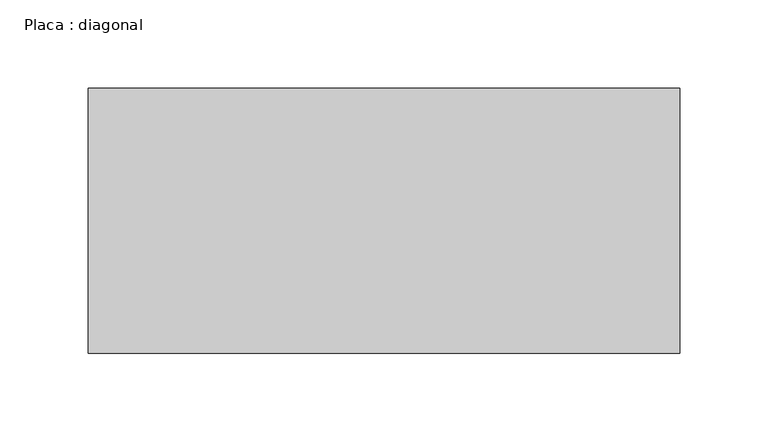
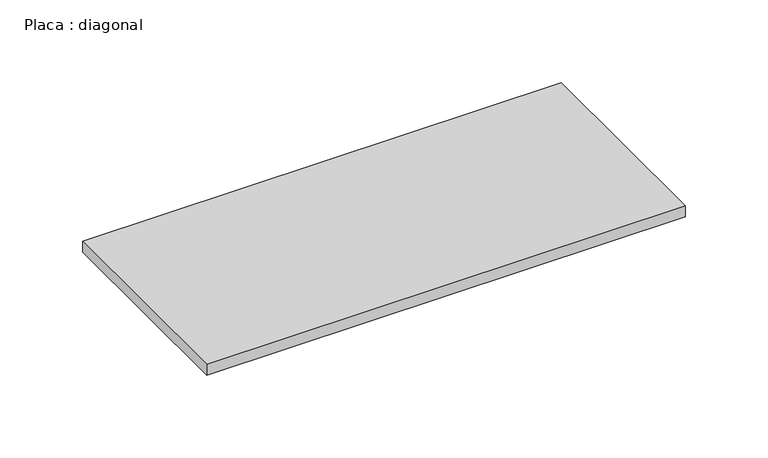
"""IFC4 building model written with IfcOpenShell, lengths in millimetres: beam geometry, Placa : diagonal."""

import ifcopenshell
import ifcopenshell.guid

model = None  # the IFC model being written
_history = None  # IfcOwnerHistory: only IFC2X3 demands one
_inside = {}  # id of a spatial element -> (the spatial element, [elements in it])
_under = {}  # id of a project, library or spatial element -> (it, [spatial elements below it])
_declared = {}  # id of a project -> (the project, [libraries it declares])
_typed = {}  # id of a type object -> (the type object, [elements of that type])
_made_of = {}  # id of a material, layer set ... -> (it, [elements and type objects made of it])


def new_model(schema):
    """Start an empty IFC model of exactly this schema.

    Asked for "IFC4X3", IfcOpenShell would pick the latest addendum, in which some entities
    have other attributes; the version numbers below select the first issue.
    IFC2X3 requires an IfcOwnerHistory on every rooted entity: one is made here for all.
    """
    global model, _history
    if schema == "IFC4X3":
        model = ifcopenshell.file(schema_version=(4, 3, 0, 0))
    else:
        model = ifcopenshell.file(schema=schema)
    _inside.clear()
    _under.clear()
    _declared.clear()
    _typed.clear()
    _made_of.clear()
    _history = None
    if model.schema == "IFC2X3":
        org = make("IfcOrganization", Name="unknown")
        user = make(
            "IfcPersonAndOrganization",
            ThePerson=make("IfcPerson", FamilyName="unknown"),
            TheOrganization=org,
        )
        app = make(
            "IfcApplication",
            ApplicationDeveloper=org,
            Version="unknown",
            ApplicationFullName="unknown",
            ApplicationIdentifier="unknown",
        )
        _history = make(
            "IfcOwnerHistory",
            OwningUser=user,
            OwningApplication=app,
            ChangeAction="ADDED",
            CreationDate=0,
        )
    return model


def make(cls, **values):
    """One entity of the class cls with the attributes given. An attribute that is None is left unset."""
    return model.create_entity(
        cls, **{name: value for name, value in values.items() if value is not None}
    )


def rooted(cls, **values):
    """An entity with a GlobalId (a new one), such as an element, a storey or a relation."""
    return make(cls, GlobalId=ifcopenshell.guid.new(), OwnerHistory=_history, **values)


def si_unit(unit_type, name, prefix=None):
    """IfcSIUnit, for example si_unit("LENGTHUNIT", "METRE", prefix="MILLI")."""
    return make("IfcSIUnit", UnitType=unit_type, Prefix=prefix, Name=name)


def assignment(units):
    """IfcUnitAssignment: the units of a project."""
    return None if units is None else make("IfcUnitAssignment", Units=units)


def point(xyz):
    """IfcCartesianPoint."""
    return None if xyz is None else make("IfcCartesianPoint", Coordinates=xyz)


def direction(xyz):
    """IfcDirection."""
    return None if xyz is None else make("IfcDirection", DirectionRatios=xyz)


def frame(location, z_axis=None, x_axis=None):
    """IfcAxis2Placement3D, a coordinate frame: its origin and axes. An axis left out is left unset."""
    return make(
        "IfcAxis2Placement3D",
        Location=point(location),
        Axis=direction(z_axis),
        RefDirection=direction(x_axis),
    )


def origin():
    """The frame at (0, 0, 0) with its axes left unset."""
    return frame((0.0, 0.0, 0.0))


def place(relative_to, where):
    """IfcLocalPlacement: puts the frame where relative to a parent placement (None: the world)."""
    return make(
        "IfcLocalPlacement", PlacementRelTo=relative_to, RelativePlacement=where
    )


def context(
    kind, dimensions, precision=None, world=None, true_north=None, identifier=None
):
    """IfcGeometricRepresentationContext, for example the 3D "Model" context."""
    return make(
        "IfcGeometricRepresentationContext",
        ContextIdentifier=identifier,
        ContextType=kind,
        CoordinateSpaceDimension=dimensions,
        Precision=precision,
        WorldCoordinateSystem=world,
        TrueNorth=true_north,
    )


def project(units=None, contexts=None):
    """IfcProject with its units and contexts."""
    return rooted(
        "IfcProject",
        Name="project",
        RepresentationContexts=contexts,
        UnitsInContext=assignment(units),
    )


def spatial(cls, under=None, at=None, **own):
    """A site, building, storey or space (cls), placed at a placement, below another one or the project."""
    s = rooted(cls, ObjectPlacement=at, **own)
    if under is not None:
        _under.setdefault(under.id(), (under, []))[1].append(s)
    return s


def polyline(points):
    """IfcPolyline through the points."""
    return make("IfcPolyline", Points=[point(p) for p in points])


def outline(outer, holes=None, kind="AREA"):
    """IfcArbitraryClosedProfileDef: a profile drawn as a closed curve; with holes, ...WithVoids."""
    if holes is None:
        return make("IfcArbitraryClosedProfileDef", ProfileType=kind, OuterCurve=outer)
    return make(
        "IfcArbitraryProfileDefWithVoids",
        ProfileType=kind,
        OuterCurve=outer,
        InnerCurves=holes,
    )


def extrude(swept, where, along, depth):
    """IfcExtrudedAreaSolid: the profile swept, set in the frame where, extruded along a direction by depth."""
    return make(
        "IfcExtrudedAreaSolid",
        SweptArea=swept,
        Position=where,
        ExtrudedDirection=direction(along),
        Depth=depth,
    )


def shape(context_of_items, identifier, shape_type, items):
    """IfcShapeRepresentation: the items that make up one representation, for example the "Body"."""
    return make(
        "IfcShapeRepresentation",
        ContextOfItems=context_of_items,
        RepresentationIdentifier=identifier,
        RepresentationType=shape_type,
        Items=items,
    )


def source(mapping_origin, context_of_items, identifier, shape_type, items):
    """IfcRepresentationMap: a shape defined once, which mapped items show again and again."""
    return make(
        "IfcRepresentationMap",
        MappingOrigin=mapping_origin,
        MappedRepresentation=shape(context_of_items, identifier, shape_type, items),
    )


def transform(
    local_origin,
    x_axis=None,
    y_axis=None,
    z_axis=None,
    scale=None,
    scale2=None,
    scale3=None,
    uniform=True,
):
    """IfcCartesianTransformationOperator3D, or its non-uniform kind. x_axis, y_axis, z_axis: its Axis1, 2, 3."""
    if uniform:
        return make(
            "IfcCartesianTransformationOperator3D",
            Axis1=direction(x_axis),
            Axis2=direction(y_axis),
            LocalOrigin=point(local_origin),
            Scale=scale,
            Axis3=direction(z_axis),
        )
    return make(
        "IfcCartesianTransformationOperator3DnonUniform",
        Axis1=direction(x_axis),
        Axis2=direction(y_axis),
        LocalOrigin=point(local_origin),
        Scale=scale,
        Axis3=direction(z_axis),
        Scale2=scale2,
        Scale3=scale3,
    )


def mapped(mapping_source, mapping_target):
    """IfcMappedItem: shows the shape of a source again, moved by a transform."""
    return make(
        "IfcMappedItem", MappingSource=mapping_source, MappingTarget=mapping_target
    )


def made_of(thing, what):
    """Note that an element or type object is made of a material, layer set ...; save() writes the relation."""
    if what is not None:
        _made_of.setdefault(what.id(), (what, []))[1].append(thing)
    return thing


def element(
    cls,
    number,
    at=None,
    inside=None,
    cuts=None,
    type_object=None,
    material=None,
    context=None,
    identifier="Body",
    shape_type=None,
    held_by="IfcProductDefinitionShape",
    body=None,
    shapes=None,
    **own,
):
    """One element of the class cls, such as IfcWall. Its Tag is "e" and its number.

    at: its placement. inside: the storey or other place that contains it. cuts: it is an
    opening in that element (IfcRelVoidsElement). A single representation is given by context,
    identifier, shape_type and body (its items); several are given by shapes. held_by: the class
    of the entity that holds the representations. save() writes the other relations.
    """
    e = rooted(cls, Tag="e%d" % number, ObjectPlacement=at, **own)
    if body is not None:
        shapes = [shape(context, identifier, shape_type, body)]
    if shapes is not None:
        e.Representation = make(held_by, Representations=shapes)
    if inside is not None:
        _inside.setdefault(inside.id(), (inside, []))[1].append(e)
    if cuts is not None:
        rooted(
            "IfcRelVoidsElement", RelatingBuildingElement=cuts, RelatedOpeningElement=e
        )
    if type_object is not None:
        _typed.setdefault(type_object.id(), (type_object, []))[1].append(e)
    return made_of(e, material)


def aggregate(whole, parts):
    """IfcRelAggregates: a whole, such as a stair, and the parts it consists of."""
    return rooted("IfcRelAggregates", RelatingObject=whole, RelatedObjects=parts)


def save(model, path):
    """Write the relations noted so far, then the file.

    IfcRelAggregates (storeys below a building ...), IfcRelContainedInSpatialStructure (elements
    in a storey), IfcRelDefinesByType, IfcRelAssociatesMaterial and IfcRelDeclares: one each for
    every whole, place, type object, material and project.
    """
    for whole, parts in _under.values():
        aggregate(whole, parts)
    for where, things in _inside.values():
        rooted(
            "IfcRelContainedInSpatialStructure",
            RelatedElements=things,
            RelatingStructure=where,
        )
    for kind, things in _typed.values():
        rooted("IfcRelDefinesByType", RelatedObjects=things, RelatingType=kind)
    for what, things in _made_of.values():
        rooted("IfcRelAssociatesMaterial", RelatedObjects=things, RelatingMaterial=what)
    for by, libraries in _declared.values():
        rooted("IfcRelDeclares", RelatingContext=by, RelatedDefinitions=libraries)
    model.write(path)


def placa_diagonal_266b1673(model_context):
    return source(origin(), model_context, "Body", "SweptSolid", [
        extrude(outline(polyline([(167.1833817, 75.0), (167.1833817, -75.0), (-167.541755, -75.0), (-167.541755, 75.0), (167.1833817, 75.0)])), frame((0.0, 0.0, -4.0), z_axis=(0.0, 0.0, 1.0), x_axis=(1.0, 0.0, 0.0)), (0.0, 0.0, 1.0), 8.0),
    ])


if __name__ == "__main__":
    model = new_model("IFC4")
    model_context = context("Model", 3, world=origin())
    ifc_project = project(units=[si_unit("LENGTHUNIT", "METRE", prefix="MILLI")], contexts=[model_context])
    site = spatial("IfcSite", under=ifc_project)
    building = spatial("IfcBuilding", under=site)
    placement = place(None, origin())
    placa_diagonal_shape = placa_diagonal_266b1673(model_context)
    element("IfcBeam", 1, ObjectType="Placa : diagonal", at=placement, inside=building, context=model_context, shape_type="MappedRepresentation", body=[
        mapped(placa_diagonal_shape, transform((0.0, 0.0, 0.0), x_axis=(1.0, 0.0, 0.0), y_axis=(0.0, 1.0, 0.0), z_axis=(0.0, 0.0, 1.0))),
    ])
    save(model, "model.ifc")

# Revit data of these elements
# Type "Placa : diagonal"
#   W = 0
#   Length [instance default] = 1.50 m
#   b = 0.15 m
#   d = 0.008 m
#   A = 0 m²
#   Structural Material [instance default] = Aço, 45-345
# Element 1 (IfcBeam, "Placa : diagonal")
#   Materials on its faces: "Aço, 45-345"
# Materials
#   "Aço, 45-345": class "Metal", colour RGB 247 247 247, transparency 0, Description = "Aço 345 MPa", Cost = 0
